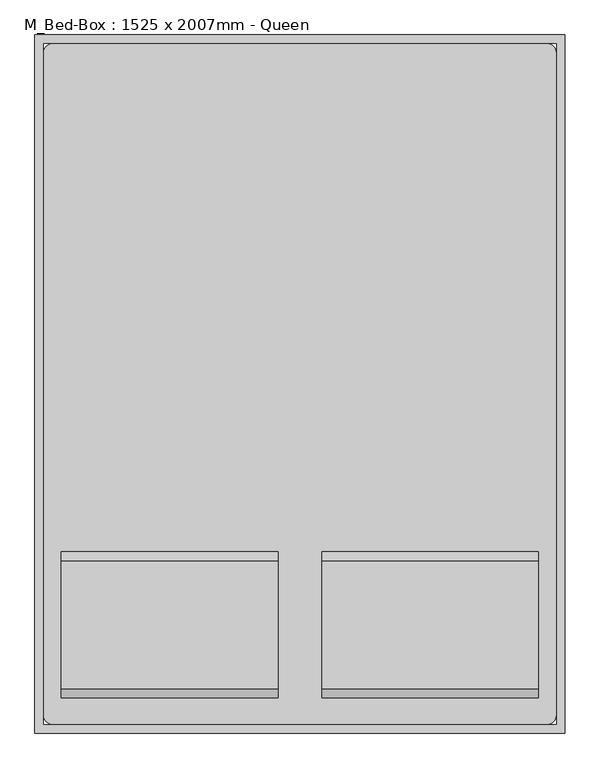
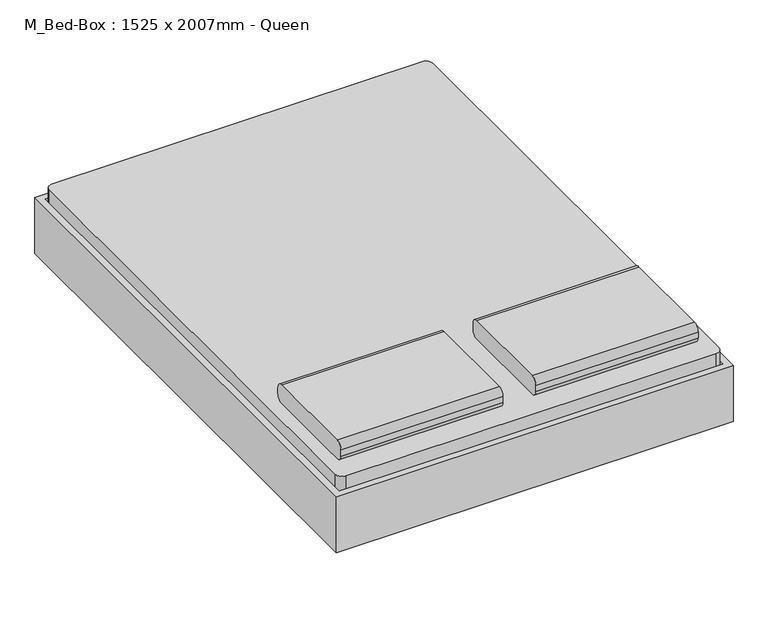
"""IFC4 building model written with IfcOpenShell, lengths in millimetres: furniture geometry, M_Bed-Box : 1525 x 2007mm - Queen."""

import ifcopenshell
import ifcopenshell.guid

model = None  # the IFC model being written
_history = None  # IfcOwnerHistory: only IFC2X3 demands one
_inside = {}  # id of a spatial element -> (the spatial element, [elements in it])
_under = {}  # id of a project, library or spatial element -> (it, [spatial elements below it])
_declared = {}  # id of a project -> (the project, [libraries it declares])
_typed = {}  # id of a type object -> (the type object, [elements of that type])
_made_of = {}  # id of a material, layer set ... -> (it, [elements and type objects made of it])


def new_model(schema):
    """Start an empty IFC model of exactly this schema.

    Asked for "IFC4X3", IfcOpenShell would pick the latest addendum, in which some entities
    have other attributes; the version numbers below select the first issue.
    IFC2X3 requires an IfcOwnerHistory on every rooted entity: one is made here for all.
    """
    global model, _history
    if schema == "IFC4X3":
        model = ifcopenshell.file(schema_version=(4, 3, 0, 0))
    else:
        model = ifcopenshell.file(schema=schema)
    _inside.clear()
    _under.clear()
    _declared.clear()
    _typed.clear()
    _made_of.clear()
    _history = None
    if model.schema == "IFC2X3":
        org = make("IfcOrganization", Name="unknown")
        user = make(
            "IfcPersonAndOrganization",
            ThePerson=make("IfcPerson", FamilyName="unknown"),
            TheOrganization=org,
        )
        app = make(
            "IfcApplication",
            ApplicationDeveloper=org,
            Version="unknown",
            ApplicationFullName="unknown",
            ApplicationIdentifier="unknown",
        )
        _history = make(
            "IfcOwnerHistory",
            OwningUser=user,
            OwningApplication=app,
            ChangeAction="ADDED",
            CreationDate=0,
        )
    return model


def make(cls, **values):
    """One entity of the class cls with the attributes given. An attribute that is None is left unset."""
    return model.create_entity(
        cls, **{name: value for name, value in values.items() if value is not None}
    )


def rooted(cls, **values):
    """An entity with a GlobalId (a new one), such as an element, a storey or a relation."""
    return make(cls, GlobalId=ifcopenshell.guid.new(), OwnerHistory=_history, **values)


def si_unit(unit_type, name, prefix=None):
    """IfcSIUnit, for example si_unit("LENGTHUNIT", "METRE", prefix="MILLI")."""
    return make("IfcSIUnit", UnitType=unit_type, Prefix=prefix, Name=name)


def assignment(units):
    """IfcUnitAssignment: the units of a project."""
    return None if units is None else make("IfcUnitAssignment", Units=units)


def point(xyz):
    """IfcCartesianPoint."""
    return None if xyz is None else make("IfcCartesianPoint", Coordinates=xyz)


def direction(xyz):
    """IfcDirection."""
    return None if xyz is None else make("IfcDirection", DirectionRatios=xyz)


def frame(location, z_axis=None, x_axis=None):
    """IfcAxis2Placement3D, a coordinate frame: its origin and axes. An axis left out is left unset."""
    return make(
        "IfcAxis2Placement3D",
        Location=point(location),
        Axis=direction(z_axis),
        RefDirection=direction(x_axis),
    )


def frame_2d(location, x_axis=None):
    """IfcAxis2Placement2D, a coordinate frame in the plane: its origin and x axis."""
    return make(
        "IfcAxis2Placement2D", Location=point(location), RefDirection=direction(x_axis)
    )


def origin():
    """The frame at (0, 0, 0) with its axes left unset."""
    return frame((0.0, 0.0, 0.0))


def place(relative_to, where):
    """IfcLocalPlacement: puts the frame where relative to a parent placement (None: the world)."""
    return make(
        "IfcLocalPlacement", PlacementRelTo=relative_to, RelativePlacement=where
    )


def context(
    kind, dimensions, precision=None, world=None, true_north=None, identifier=None
):
    """IfcGeometricRepresentationContext, for example the 3D "Model" context."""
    return make(
        "IfcGeometricRepresentationContext",
        ContextIdentifier=identifier,
        ContextType=kind,
        CoordinateSpaceDimension=dimensions,
        Precision=precision,
        WorldCoordinateSystem=world,
        TrueNorth=true_north,
    )


def project(units=None, contexts=None):
    """IfcProject with its units and contexts."""
    return rooted(
        "IfcProject",
        Name="project",
        RepresentationContexts=contexts,
        UnitsInContext=assignment(units),
    )


def spatial(cls, under=None, at=None, **own):
    """A site, building, storey or space (cls), placed at a placement, below another one or the project."""
    s = rooted(cls, ObjectPlacement=at, **own)
    if under is not None:
        _under.setdefault(under.id(), (under, []))[1].append(s)
    return s


def polyline(points):
    """IfcPolyline through the points."""
    return make("IfcPolyline", Points=[point(p) for p in points])


def circle_curve(where, radius):
    """IfcCircle in the frame where."""
    return make("IfcCircle", Position=where, Radius=radius)


def trimmed(basis, trim1, trim2, sense, master):
    """IfcTrimmedCurve: the piece of a basis curve between two trims."""
    return make(
        "IfcTrimmedCurve",
        BasisCurve=basis,
        Trim1=trim1,
        Trim2=trim2,
        SenseAgreement=sense,
        MasterRepresentation=master,
    )


def segment(curve, same_sense, transition):
    """IfcCompositeCurveSegment."""
    return make(
        "IfcCompositeCurveSegment",
        Transition=transition,
        SameSense=same_sense,
        ParentCurve=curve,
    )


def composite_curve(segments, self_intersect=None):
    """IfcCompositeCurve: segments joined end to end."""
    return make("IfcCompositeCurve", Segments=segments, SelfIntersect=self_intersect)


def outline(outer, holes=None, kind="AREA"):
    """IfcArbitraryClosedProfileDef: a profile drawn as a closed curve; with holes, ...WithVoids."""
    if holes is None:
        return make("IfcArbitraryClosedProfileDef", ProfileType=kind, OuterCurve=outer)
    return make(
        "IfcArbitraryProfileDefWithVoids",
        ProfileType=kind,
        OuterCurve=outer,
        InnerCurves=holes,
    )


def extrude(swept, where, along, depth):
    """IfcExtrudedAreaSolid: the profile swept, set in the frame where, extruded along a direction by depth."""
    return make(
        "IfcExtrudedAreaSolid",
        SweptArea=swept,
        Position=where,
        ExtrudedDirection=direction(along),
        Depth=depth,
    )


def shape(context_of_items, identifier, shape_type, items):
    """IfcShapeRepresentation: the items that make up one representation, for example the "Body"."""
    return make(
        "IfcShapeRepresentation",
        ContextOfItems=context_of_items,
        RepresentationIdentifier=identifier,
        RepresentationType=shape_type,
        Items=items,
    )


def source(mapping_origin, context_of_items, identifier, shape_type, items):
    """IfcRepresentationMap: a shape defined once, which mapped items show again and again."""
    return make(
        "IfcRepresentationMap",
        MappingOrigin=mapping_origin,
        MappedRepresentation=shape(context_of_items, identifier, shape_type, items),
    )


def transform(
    local_origin,
    x_axis=None,
    y_axis=None,
    z_axis=None,
    scale=None,
    scale2=None,
    scale3=None,
    uniform=True,
):
    """IfcCartesianTransformationOperator3D, or its non-uniform kind. x_axis, y_axis, z_axis: its Axis1, 2, 3."""
    if uniform:
        return make(
            "IfcCartesianTransformationOperator3D",
            Axis1=direction(x_axis),
            Axis2=direction(y_axis),
            LocalOrigin=point(local_origin),
            Scale=scale,
            Axis3=direction(z_axis),
        )
    return make(
        "IfcCartesianTransformationOperator3DnonUniform",
        Axis1=direction(x_axis),
        Axis2=direction(y_axis),
        LocalOrigin=point(local_origin),
        Scale=scale,
        Axis3=direction(z_axis),
        Scale2=scale2,
        Scale3=scale3,
    )


def mapped(mapping_source, mapping_target):
    """IfcMappedItem: shows the shape of a source again, moved by a transform."""
    return make(
        "IfcMappedItem", MappingSource=mapping_source, MappingTarget=mapping_target
    )


def made_of(thing, what):
    """Note that an element or type object is made of a material, layer set ...; save() writes the relation."""
    if what is not None:
        _made_of.setdefault(what.id(), (what, []))[1].append(thing)
    return thing


def element(
    cls,
    number,
    at=None,
    inside=None,
    cuts=None,
    type_object=None,
    material=None,
    context=None,
    identifier="Body",
    shape_type=None,
    held_by="IfcProductDefinitionShape",
    body=None,
    shapes=None,
    **own,
):
    """One element of the class cls, such as IfcWall. Its Tag is "e" and its number.

    at: its placement. inside: the storey or other place that contains it. cuts: it is an
    opening in that element (IfcRelVoidsElement). A single representation is given by context,
    identifier, shape_type and body (its items); several are given by shapes. held_by: the class
    of the entity that holds the representations. save() writes the other relations.
    """
    e = rooted(cls, Tag="e%d" % number, ObjectPlacement=at, **own)
    if body is not None:
        shapes = [shape(context, identifier, shape_type, body)]
    if shapes is not None:
        e.Representation = make(held_by, Representations=shapes)
    if inside is not None:
        _inside.setdefault(inside.id(), (inside, []))[1].append(e)
    if cuts is not None:
        rooted(
            "IfcRelVoidsElement", RelatingBuildingElement=cuts, RelatedOpeningElement=e
        )
    if type_object is not None:
        _typed.setdefault(type_object.id(), (type_object, []))[1].append(e)
    return made_of(e, material)


def aggregate(whole, parts):
    """IfcRelAggregates: a whole, such as a stair, and the parts it consists of."""
    return rooted("IfcRelAggregates", RelatingObject=whole, RelatedObjects=parts)


def save(model, path):
    """Write the relations noted so far, then the file.

    IfcRelAggregates (storeys below a building ...), IfcRelContainedInSpatialStructure (elements
    in a storey), IfcRelDefinesByType, IfcRelAssociatesMaterial and IfcRelDeclares: one each for
    every whole, place, type object, material and project.
    """
    for whole, parts in _under.values():
        aggregate(whole, parts)
    for where, things in _inside.values():
        rooted(
            "IfcRelContainedInSpatialStructure",
            RelatedElements=things,
            RelatingStructure=where,
        )
    for kind, things in _typed.values():
        rooted("IfcRelDefinesByType", RelatedObjects=things, RelatingType=kind)
    for what, things in _made_of.values():
        rooted("IfcRelAssociatesMaterial", RelatedObjects=things, RelatingMaterial=what)
    for by, libraries in _declared.values():
        rooted("IfcRelDeclares", RelatingContext=by, RelatedDefinitions=libraries)
    model.write(path)


def plane_surface(at):
    """IfcPlane: the flat surface through the origin of the frame at, square to its z axis."""
    return make("IfcPlane", Position=at)


def cylinder_surface(at, radius):
    """IfcCylindricalSurface: all points at the distance radius from the z axis of the frame at."""
    return make("IfcCylindricalSurface", Position=at, Radius=radius)


def revolved_surface(curve, axis_point, axis_direction):
    """IfcSurfaceOfRevolution: the curve turned about the line through axis_point along axis_direction."""
    return make(
        "IfcSurfaceOfRevolution",
        SweptCurve=make("IfcArbitraryOpenProfileDef", ProfileType="CURVE", Curve=curve),
        AxisPosition=make("IfcAxis1Placement", Location=point(axis_point), Axis=direction(axis_direction)),
    )


def advanced_brep(points, edges, surfaces, faces):
    """IfcAdvancedBrep: a solid bounded by faces that lie on surfaces and meet in shared edges.

    An edge is (start, end): straight between two places in points (the first is 0);
    or (start, end, curve); or (start, end, curve, False) where it runs against its curve.
    A face is (place in surfaces, loops), or (place, loops, False) where it looks against
    its surface's normal. A loop lists edges by number (the first is 1), with a minus sign
    where the edge is run from its end to its start. The first loop is the outer one.
    """
    corners = [point(p) for p in points]
    vertices = [make("IfcVertexPoint", VertexGeometry=c) for c in corners]
    made = []
    for start, end, *more in edges:
        made.append(
            make(
                "IfcEdgeCurve",
                EdgeStart=vertices[start],
                EdgeEnd=vertices[end],
                EdgeGeometry=more[0] if more else make("IfcPolyline", Points=[corners[start], corners[end]]),
                SameSense=more[1] if len(more) > 1 else True,
            )
        )
    hull = []
    for where, loops, *sense in faces:
        bounds = []
        for j, loop in enumerate(loops):
            ring = [make("IfcOrientedEdge", EdgeElement=made[abs(k) - 1], Orientation=k > 0) for k in loop]
            bounds.append(
                make(
                    "IfcFaceOuterBound" if j == 0 else "IfcFaceBound",
                    Bound=make("IfcEdgeLoop", EdgeList=ring),
                    Orientation=True,
                )
            )
        hull.append(make("IfcAdvancedFace", Bounds=bounds, FaceSurface=surfaces[where], SameSense=sense[0] if sense else True))
    return make("IfcAdvancedBrep", Outer=make("IfcClosedShell", CfsFaces=hull))


def m_bed_box_1525_x_2007mm_queen_6710bf5b(model_context):
    return source(origin(), model_context, "Body", "SolidModel", [
        extrude(outline(composite_curve([segment(trimmed(circle_curve(frame_2d((-642.0704918, 431.8)), 25.4), [point((-642.0704918, 406.4))], [point((-667.4704918, 431.8))], False, "CARTESIAN"), True, "CONTINUOUS"), segment(polyline([(-667.4704918, 431.8), (-667.4704918, 457.2)]), True, "CONTINUOUS"), segment(trimmed(circle_curve(frame_2d((-642.0704918, 457.2)), 25.4), [point((-667.4704918, 457.2))], [point((-642.0704918, 482.6))], False, "CARTESIAN"), True, "CONTINUOUS"), segment(polyline([(-642.0704918, 482.6), (-273.7704918, 482.6)]), True, "CONTINUOUS"), segment(trimmed(circle_curve(frame_2d((-273.7704918, 457.2)), 25.4), [point((-273.7704918, 482.6))], [point((-248.3704918, 457.2))], False, "CARTESIAN"), True, "CONTINUOUS"), segment(polyline([(-248.3704918, 457.2), (-248.3704918, 431.8)]), True, "CONTINUOUS"), segment(trimmed(circle_curve(frame_2d((-273.7704918, 431.8)), 25.4), [point((-248.3704918, 431.8))], [point((-273.7704918, 406.4))], False, "CARTESIAN"), True, "CONTINUOUS"), segment(polyline([(-273.7704918, 406.4), (-642.0704918, 406.4)]), True, "CONTINUOUS")], self_intersect=False)), frame((402.652459, 0.0, 0.0), z_axis=(1.0, 0.0, 0.0), x_axis=(0.0, 1.0, 0.0)), (0.0, 0.0, 1.0), 622.8),
        extrude(outline(composite_curve([segment(trimmed(circle_curve(frame_2d((-642.0704918, 431.8)), 25.4), [point((-642.0704918, 406.4))], [point((-667.4704918, 431.8))], False, "CARTESIAN"), True, "CONTINUOUS"), segment(polyline([(-667.4704918, 431.8), (-667.4704918, 457.2)]), True, "CONTINUOUS"), segment(trimmed(circle_curve(frame_2d((-642.0704918, 457.2)), 25.4), [point((-667.4704918, 457.2))], [point((-642.0704918, 482.6))], False, "CARTESIAN"), True, "CONTINUOUS"), segment(polyline([(-642.0704918, 482.6), (-273.7704918, 482.6)]), True, "CONTINUOUS"), segment(trimmed(circle_curve(frame_2d((-273.7704918, 457.2)), 25.4), [point((-273.7704918, 482.6))], [point((-248.3704918, 457.2))], False, "CARTESIAN"), True, "CONTINUOUS"), segment(polyline([(-248.3704918, 457.2), (-248.3704918, 431.8)]), True, "CONTINUOUS"), segment(trimmed(circle_curve(frame_2d((-273.7704918, 431.8)), 25.4), [point((-248.3704918, 431.8))], [point((-273.7704918, 406.4))], False, "CARTESIAN"), True, "CONTINUOUS"), segment(polyline([(-273.7704918, 406.4), (-642.0704918, 406.4)]), True, "CONTINUOUS")], self_intersect=False)), frame((-347.147541, 0.0, 0.0), z_axis=(1.0, 0.0, 0.0), x_axis=(0.0, 1.0, 0.0)), (0.0, 0.0, 1.0), 622.8),
        advanced_brep(
        [(-397.6231784, -515.0704918, 177.8), (-397.6231784, -515.0704918, 196.85), (-397.6231784, -438.8704918, 196.85), (-397.6231784, -438.8704918, 177.8), (-346.8231784, -438.8704918, 177.8), (-346.8231784, -515.0704918, 177.8), (-334.6869899, -438.8704918, 196.85), (-334.6869899, -515.0704918, 196.85), (-270.7523099, -438.8704918, 14.6654962), (-270.7523099, -515.0704918, 14.6654962), (-253.4871466, -438.8704918, 22.716374), (-253.4871466, -515.0704918, 22.716374), (-247.7320921, -438.8704918, 0.0), (-247.7320921, -515.0704918, 0.0), (-247.7320921, -438.8704918, 19.05), (-247.7320921, -515.0704918, 19.05), (-169.1195862, -438.8704918, 0.0), (-169.1195862, -515.0704918, 0.0), (-169.1195862, -438.8704918, 19.05), (-169.1195862, -515.0704918, 19.05), (-156.4195862, -438.8704918, 3.4029547), (-156.4195862, -515.0704918, 3.4029547), (-165.9445862, -438.8704918, 19.9007387), (-165.9445862, -515.0704918, 19.9007387), (-96.322541, -438.8704918, 38.1), (-96.322541, -515.0704918, 38.1), (-101.4269731, -438.8704918, 57.15), (-101.4269731, -515.0704918, 57.15), (774.9518216, -438.8704918, 38.1), (774.9518216, -515.0704918, 38.1), (780.0562537, -438.8704918, 57.15), (780.0562537, -515.0704918, 57.15), (835.0488669, -438.8704918, 3.4029547), (835.0488669, -515.0704918, 3.4029547), (844.5738669, -438.8704918, 19.9007387), (844.5738669, -515.0704918, 19.9007387), (847.7488669, -438.8704918, 0.0), (847.7488669, -515.0704918, 0.0), (847.7488669, -438.8704918, 19.05), (847.7488669, -515.0704918, 19.05), (926.3613728, -438.8704918, 0.0), (926.3613728, -515.0704918, 0.0), (926.3613728, -438.8704918, 19.05), (926.3613728, -515.0704918, 19.05), (949.3815906, -438.8704918, 14.6654962), (949.3815906, -515.0704918, 14.6654962), (932.1164272, -438.8704918, 22.716374), (932.1164272, -515.0704918, 22.716374), (1025.452459, -438.8704918, 177.8), (1025.452459, -515.0704918, 177.8), (1013.3162705, -438.8704918, 196.85), (1013.3162705, -515.0704918, 196.85), (1076.252459, -515.0704918, 177.8), (1076.252459, -438.8704918, 177.8), (1076.252459, -438.8704918, 196.85), (1076.252459, -515.0704918, 196.85)],
        [
            (0, 1),
            (1, 2),
            (2, 3),
            (3, 0),
            (3, 4),
            (4, 5),
            (5, 0),
            (2, 6),
            (6, 4),
            (1, 7),
            (7, 6),
            (5, 7),
            (4, 8),
            (8, 9),
            (9, 5),
            (6, 10),
            (10, 8),
            (7, 11),
            (11, 10),
            (9, 11),
            (12, 13),
            (13, 9, circle_curve(frame((-247.7320921, -515.0704918, 25.4), z_axis=(0.0, 1.0, 0.0), x_axis=(-0.906307787036649, 0.0, -0.4226182617407015)), 25.4)),
            (8, 12, circle_curve(frame((-247.7320921, -438.8704918, 25.4), z_axis=(0.0, -1.0, 0.0), x_axis=(-0.906307787036649, 0.0, -0.4226182617407015)), 25.4)),
            (14, 12),
            (10, 14, circle_curve(frame((-247.7320921, -438.8704918, 25.4), z_axis=(0.0, -1.0, 0.0), x_axis=(-0.906307787036649, 0.0, -0.4226182617407015)), 6.35)),
            (15, 14),
            (11, 15, circle_curve(frame((-247.7320921, -515.0704918, 25.4), z_axis=(0.0, -1.0, 0.0), x_axis=(-0.906307787036649, 0.0, -0.4226182617407015)), 6.35)),
            (13, 15),
            (12, 16),
            (16, 17),
            (17, 13),
            (14, 18),
            (18, 16),
            (15, 19),
            (19, 18),
            (17, 19),
            (20, 21),
            (21, 17, circle_curve(frame((-169.1195862, -515.0704918, 25.4), z_axis=(0.0, 1.0, 0.0), x_axis=(0.0, 0.0, -1.0)), 25.4)),
            (16, 20, circle_curve(frame((-169.1195862, -438.8704918, 25.4), z_axis=(0.0, -1.0, 0.0), x_axis=(0.0, 0.0, -1.0)), 25.4)),
            (22, 20),
            (18, 22, circle_curve(frame((-169.1195862, -438.8704918, 25.4), z_axis=(0.0, -1.0, 0.0), x_axis=(0.0, 0.0, -1.0)), 6.35)),
            (23, 22),
            (19, 23, circle_curve(frame((-169.1195862, -515.0704918, 25.4), z_axis=(0.0, -1.0, 0.0), x_axis=(0.0, 0.0, -1.0)), 6.35)),
            (21, 23),
            (20, 24),
            (24, 25),
            (25, 21),
            (22, 26),
            (26, 24),
            (23, 27),
            (27, 26),
            (25, 27),
            (24, 28),
            (28, 29),
            (29, 25),
            (26, 30),
            (30, 28),
            (27, 31),
            (31, 30),
            (29, 31),
            (28, 32),
            (32, 33),
            (33, 29),
            (30, 34),
            (34, 32),
            (31, 35),
            (35, 34),
            (33, 35),
            (36, 37),
            (37, 33, circle_curve(frame((847.7488669, -515.0704918, 25.4), z_axis=(0.0, 1.0, 0.0), x_axis=(-0.5000000000000463, 0.0, -0.8660254037844118)), 25.4)),
            (32, 36, circle_curve(frame((847.7488669, -438.8704918, 25.4), z_axis=(0.0, -1.0, 0.0), x_axis=(-0.5000000000000463, 0.0, -0.8660254037844118)), 25.4)),
            (38, 36),
            (34, 38, circle_curve(frame((847.7488669, -438.8704918, 25.4), z_axis=(0.0, -1.0, 0.0), x_axis=(-0.5000000000000463, 0.0, -0.8660254037844118)), 6.35)),
            (39, 38),
            (35, 39, circle_curve(frame((847.7488669, -515.0704918, 25.4), z_axis=(0.0, -1.0, 0.0), x_axis=(-0.5000000000000463, 0.0, -0.8660254037844118)), 6.35)),
            (37, 39),
            (36, 40),
            (40, 41),
            (41, 37),
            (38, 42),
            (42, 40),
            (39, 43),
            (43, 42),
            (41, 43),
            (44, 45),
            (45, 41, circle_curve(frame((926.3613728, -515.0704918, 25.4), z_axis=(0.0, 1.0, 0.0), x_axis=(0.0, 0.0, -1.0)), 25.4)),
            (40, 44, circle_curve(frame((926.3613728, -438.8704918, 25.4), z_axis=(0.0, -1.0, 0.0), x_axis=(0.0, 0.0, -1.0)), 25.4)),
            (46, 44),
            (42, 46, circle_curve(frame((926.3613728, -438.8704918, 25.4), z_axis=(0.0, -1.0, 0.0), x_axis=(0.0, 0.0, -1.0)), 6.35)),
            (47, 46),
            (43, 47, circle_curve(frame((926.3613728, -515.0704918, 25.4), z_axis=(0.0, -1.0, 0.0), x_axis=(0.0, 0.0, -1.0)), 6.35)),
            (45, 47),
            (44, 48),
            (48, 49),
            (49, 45),
            (46, 50),
            (50, 48),
            (47, 51),
            (51, 50),
            (49, 51),
            (52, 53),
            (53, 54),
            (54, 55),
            (55, 52),
            (48, 53),
            (52, 49),
            (50, 54),
            (51, 55),
        ],
        [
            plane_surface(frame((-397.6231784, -769.0704918, -152.9490627), z_axis=(-1.0, 0.0, 0.0), x_axis=(0.0, -1.0, 0.0))),
            plane_surface(frame((-397.6231784, -515.0704918, 177.8), z_axis=(0.0, 0.0, -1.0), x_axis=(1.0, 0.0, 0.0))),
            plane_surface(frame((-397.6231784, -438.8704918, 177.8), z_axis=(0.0, 1.0, 0.0), x_axis=(1.0, 0.0, 0.0))),
            plane_surface(frame((-397.6231784, -438.8704918, 196.85), z_axis=(0.0, 0.0, 1.0), x_axis=(1.0, 0.0, 0.0))),
            plane_surface(frame((-397.6231784, -515.0704918, 196.85), z_axis=(0.0, -1.0, 0.0), x_axis=(1.0, 0.0, 0.0))),
            plane_surface(frame((-346.8231784, -515.0704918, 177.8), z_axis=(-0.9063077870366485, 0.0, -0.4226182617407029), x_axis=(0.4226182617407029, 0.0, -0.9063077870366485))),
            plane_surface(frame((-346.8231784, -438.8704918, 177.8), z_axis=(0.0, 1.0, 0.0), x_axis=(0.42261826174070266, 0.0, -0.9063077870366485))),
            plane_surface(frame((-334.6869899, -438.8704918, 196.85), z_axis=(0.9063077870366486, 0.0, 0.4226182617407026), x_axis=(0.4226182617407026, 0.0, -0.9063077870366486))),
            plane_surface(frame((-334.6869899, -515.0704918, 196.85), z_axis=(0.0, -1.0, 0.0), x_axis=(0.42261826174070266, 0.0, -0.9063077870366485))),
            cylinder_surface(frame((-247.7320921, -769.0704918, 25.4), z_axis=(0.0, 1.0, 0.0), x_axis=(-0.906307787036649, 0.0, -0.4226182617407015)), 25.4),
            plane_surface(frame((-247.7320921, -438.8704918, 25.4), z_axis=(0.0, 1.0, 0.0), x_axis=(-0.906307787036649, 0.0, -0.4226182617407015))),
            revolved_surface(polyline([(-253.4871465476827, -438.8704918, 22.716374037946544), (-253.4871465476827, -515.0704918, 22.716374037946544)]), (-247.7320921, -769.0704918, 25.4), (0.0, 1.0, 0.0)),
            plane_surface(frame((-247.7320921, -515.0704918, 25.4), z_axis=(0.0, -1.0, 0.0), x_axis=(-0.906307787036649, 0.0, -0.4226182617407015))),
            plane_surface(frame((-247.7320921, -515.0704918, 0.0), z_axis=(0.0, 0.0, -1.0), x_axis=(1.0, 0.0, 0.0))),
            plane_surface(frame((-247.7320921, -438.8704918, 0.0), z_axis=(0.0, 1.0, 0.0), x_axis=(1.0, 0.0, 0.0))),
            plane_surface(frame((-247.7320921, -438.8704918, 19.05), z_axis=(0.0, 0.0, 1.0), x_axis=(1.0, 0.0, 0.0))),
            plane_surface(frame((-247.7320921, -515.0704918, 19.05), z_axis=(0.0, -1.0, 0.0), x_axis=(1.0, 0.0, 0.0))),
            cylinder_surface(frame((-169.1195862, -769.0704918, 25.4), z_axis=(0.0, 1.0, 0.0), x_axis=(0.0, 0.0, -1.0)), 25.4),
            plane_surface(frame((-169.1195862, -438.8704918, 25.4), z_axis=(0.0, 1.0, 0.0), x_axis=(0.0, 0.0, -1.0))),
            revolved_surface(polyline([(-169.1195862, -438.8704918, 19.049999999999997), (-169.1195862, -515.0704918, 19.049999999999997)]), (-169.1195862, -769.0704918, 25.4), (0.0, 1.0, 0.0)),
            plane_surface(frame((-169.1195862, -515.0704918, 25.4), z_axis=(0.0, -1.0, 0.0), x_axis=(0.0, 0.0, -1.0))),
            plane_surface(frame((-156.4195862, -515.0704918, 3.4029547), z_axis=(0.49999999999987765, 0.0, -0.8660254037845093), x_axis=(0.8660254037845093, 0.0, 0.49999999999987765))),
            plane_surface(frame((-156.4195862, -438.8704918, 3.4029547), z_axis=(0.0, 1.0, 0.0), x_axis=(0.8660254037845091, 0.0, 0.499999999999878))),
            plane_surface(frame((-165.9445862, -438.8704918, 19.9007387), z_axis=(-0.49999999999987765, 0.0, 0.8660254037845093), x_axis=(0.8660254037845093, 0.0, 0.49999999999987765))),
            plane_surface(frame((-165.9445862, -515.0704918, 19.9007387), z_axis=(0.0, -1.0000000000000002, 0.0), x_axis=(0.8660254037845089, 0.0, 0.4999999999998785))),
            plane_surface(frame((-96.322541, -515.0704918, 38.1), z_axis=(0.0, 0.0, -1.0), x_axis=(1.0, 0.0, 0.0))),
            plane_surface(frame((-96.322541, -438.8704918, 38.1), z_axis=(0.0, 1.0, 0.0), x_axis=(1.0, 0.0, 0.0))),
            plane_surface(frame((-101.4269731, -438.8704918, 57.15), z_axis=(0.0, 0.0, 1.0), x_axis=(1.0, 0.0, 0.0))),
            plane_surface(frame((-101.4269731, -515.0704918, 57.15), z_axis=(0.0, -1.0, 0.0), x_axis=(1.0, 0.0, 0.0))),
            plane_surface(frame((774.9518216, -515.0704918, 38.1), z_axis=(-0.5000000000000452, 0.0, -0.8660254037844126), x_axis=(0.8660254037844126, 0.0, -0.5000000000000452))),
            plane_surface(frame((774.9518216, -438.8704918, 38.1), z_axis=(0.0, 1.0, 0.0), x_axis=(0.8660254037844124, 0.0, -0.5000000000000455))),
            plane_surface(frame((780.0562537, -438.8704918, 57.15), z_axis=(0.5000000000000464, 0.0, 0.8660254037844118), x_axis=(0.8660254037844118, 0.0, -0.5000000000000464))),
            plane_surface(frame((780.0562537, -515.0704918, 57.15), z_axis=(0.0, -1.0000000000000002, 0.0), x_axis=(0.866025403784413, 0.0, -0.5000000000000447))),
            cylinder_surface(frame((847.7488669, -769.0704918, 25.4), z_axis=(0.0, 1.0, 0.0), x_axis=(-0.5000000000000463, 0.0, -0.8660254037844118)), 25.4),
            plane_surface(frame((847.7488669, -438.8704918, 25.4), z_axis=(0.0, 1.0000000000000002, 0.0), x_axis=(-0.5000000000000464, 0.0, -0.866025403784412))),
            revolved_surface(polyline([(844.5738668999998, -438.8704918, 19.90073868596898), (844.5738668999998, -515.0704918, 19.90073868596898)]), (847.7488669, -769.0704918, 25.4), (0.0, 1.0, 0.0)),
            plane_surface(frame((847.7488669, -515.0704918, 25.4), z_axis=(0.0, -1.0000000000000002, 0.0), x_axis=(-0.5000000000000464, 0.0, -0.866025403784412))),
            plane_surface(frame((847.7488669, -515.0704918, 0.0), z_axis=(0.0, 0.0, -1.0), x_axis=(1.0, 0.0, 0.0))),
            plane_surface(frame((847.7488669, -438.8704918, 0.0), z_axis=(0.0, 1.0, 0.0), x_axis=(1.0, 0.0, 0.0))),
            plane_surface(frame((847.7488669, -438.8704918, 19.05), z_axis=(0.0, 0.0, 1.0), x_axis=(1.0, 0.0, 0.0))),
            plane_surface(frame((847.7488669, -515.0704918, 19.05), z_axis=(0.0, -1.0, 0.0), x_axis=(1.0, 0.0, 0.0))),
            cylinder_surface(frame((926.3613728, -769.0704918, 25.4), z_axis=(0.0, 1.0, 0.0), x_axis=(0.0, 0.0, -1.0)), 25.4),
            plane_surface(frame((926.3613728, -438.8704918, 25.4), z_axis=(0.0, 1.0, 0.0), x_axis=(0.0, 0.0, -1.0))),
            revolved_surface(polyline([(926.3613728, -438.8704918, 19.049999999999997), (926.3613728, -515.0704918, 19.049999999999997)]), (926.3613728, -769.0704918, 25.4), (0.0, 1.0, 0.0)),
            plane_surface(frame((926.3613728, -515.0704918, 25.4), z_axis=(0.0, -1.0, 0.0), x_axis=(0.0, 0.0, -1.0))),
            plane_surface(frame((949.3815906, -515.0704918, 14.6654962), z_axis=(0.9063077870366805, 0.0, -0.422618261740634), x_axis=(0.422618261740634, 0.0, 0.9063077870366805))),
            plane_surface(frame((949.3815906, -438.8704918, 14.6654962), z_axis=(0.0, 1.0, 0.0), x_axis=(0.4226182617406339, 0.0, 0.9063077870366806))),
            plane_surface(frame((932.1164272, -438.8704918, 22.716374), z_axis=(-0.9063077870366808, 0.0, 0.4226182617406335), x_axis=(0.4226182617406335, 0.0, 0.9063077870366808))),
            plane_surface(frame((932.1164272, -515.0704918, 22.716374), z_axis=(0.0, -1.0, 0.0), x_axis=(0.42261826174063294, 0.0, 0.906307787036681))),
            plane_surface(frame((1076.252459, -769.0704918, -152.9490627), z_axis=(1.0, 0.0, 0.0), x_axis=(0.0, -1.0, 0.0))),
            plane_surface(frame((1025.452459, -515.0704918, 177.8), z_axis=(0.0, 0.0, -1.0), x_axis=(1.0, 0.0, 0.0))),
            plane_surface(frame((1025.452459, -438.8704918, 177.8), z_axis=(0.0, 1.0, 0.0), x_axis=(1.0, 0.0, 0.0))),
            plane_surface(frame((1013.3162705, -438.8704918, 196.85), z_axis=(0.0, 0.0, 1.0), x_axis=(1.0, 0.0, 0.0))),
            plane_surface(frame((1013.3162705, -515.0704918, 196.85), z_axis=(0.0, -1.0, 0.0), x_axis=(1.0, 0.0, 0.0))),
        ],
        [
            (0, [[1, 2, 3, 4]]),
            (1, [[5, 6, 7, -4]]),
            (2, [[8, 9, -5, -3]]),
            (3, [[10, 11, -8, -2]]),
            (4, [[-7, 12, -10, -1]]),
            (5, [[13, 14, 15, -6]]),
            (6, [[16, 17, -13, -9]]),
            (7, [[18, 19, -16, -11]]),
            (8, [[-15, 20, -18, -12]]),
            (9, [[21, 22, -14, 23]]),
            (10, [[24, -23, -17, 25]]),
            (11, [[26, -25, -19, 27]]),
            (12, [[28, -27, -20, -22]]),
            (13, [[29, 30, 31, -21]]),
            (14, [[32, 33, -29, -24]]),
            (15, [[34, 35, -32, -26]]),
            (16, [[-31, 36, -34, -28]]),
            (17, [[37, 38, -30, 39]]),
            (18, [[40, -39, -33, 41]]),
            (19, [[42, -41, -35, 43]]),
            (20, [[44, -43, -36, -38]]),
            (21, [[45, 46, 47, -37]]),
            (22, [[48, 49, -45, -40]]),
            (23, [[50, 51, -48, -42]]),
            (24, [[-47, 52, -50, -44]]),
            (25, [[53, 54, 55, -46]]),
            (26, [[56, 57, -53, -49]]),
            (27, [[58, 59, -56, -51]]),
            (28, [[-55, 60, -58, -52]]),
            (29, [[61, 62, 63, -54]]),
            (30, [[64, 65, -61, -57]]),
            (31, [[66, 67, -64, -59]]),
            (32, [[-63, 68, -66, -60]]),
            (33, [[69, 70, -62, 71]]),
            (34, [[72, -71, -65, 73]]),
            (35, [[74, -73, -67, 75]]),
            (36, [[76, -75, -68, -70]]),
            (37, [[77, 78, 79, -69]]),
            (38, [[80, 81, -77, -72]]),
            (39, [[82, 83, -80, -74]]),
            (40, [[-79, 84, -82, -76]]),
            (41, [[85, 86, -78, 87]]),
            (42, [[88, -87, -81, 89]]),
            (43, [[90, -89, -83, 91]]),
            (44, [[92, -91, -84, -86]]),
            (45, [[93, 94, 95, -85]]),
            (46, [[96, 97, -93, -88]]),
            (47, [[98, 99, -96, -90]]),
            (48, [[-95, 100, -98, -92]]),
            (49, [[101, 102, 103, 104]]),
            (50, [[105, -101, 106, -94]]),
            (51, [[107, -102, -105, -97]]),
            (52, [[108, -103, -107, -99]]),
            (53, [[-106, -104, -108, -100]]),
        ],
    ),
        extrude(outline(composite_curve([segment(trimmed(circle_curve(frame_2d((-372.547541, -718.2704918)), 25.4), [point((-372.547541, -743.6704918))], [point((-397.947541, -718.2704918))], False, "CARTESIAN"), True, "CONTINUOUS"), segment(polyline([(-397.947541, -718.2704918), (-397.947541, 1187.1295082)]), True, "CONTINUOUS"), segment(trimmed(circle_curve(frame_2d((-372.547541, 1187.1295082)), 25.4), [point((-397.947541, 1187.1295082))], [point((-372.547541, 1212.5295082))], False, "CARTESIAN"), True, "CONTINUOUS"), segment(polyline([(-372.547541, 1212.5295082), (1050.852459, 1212.5295082)]), True, "CONTINUOUS"), segment(trimmed(circle_curve(frame_2d((1050.852459, 1187.1295082)), 25.4), [point((1050.852459, 1212.5295082))], [point((1076.252459, 1187.1295082))], False, "CARTESIAN"), True, "CONTINUOUS"), segment(polyline([(1076.252459, 1187.1295082), (1076.252459, -718.2704918)]), True, "CONTINUOUS"), segment(trimmed(circle_curve(frame_2d((1050.852459, -718.2704918)), 25.4), [point((1076.252459, -718.2704918))], [point((1050.852459, -743.6704918))], False, "CARTESIAN"), True, "CONTINUOUS"), segment(polyline([(1050.852459, -743.6704918), (-372.547541, -743.6704918)]), True, "CONTINUOUS")], self_intersect=False)), frame((0.0, 0.0, 203.2), z_axis=(0.0, 0.0, 1.0), x_axis=(1.0, 0.0, 0.0)), (0.0, 0.0, 1.0), 203.2),
        advanced_brep(
        [(-397.947541, 933.1295082, 196.85), (-397.947541, 1009.3295082, 196.85), (-397.947541, 1009.3295082, 177.8), (-397.947541, 933.1295082, 177.8), (-347.147541, 933.1295082, 177.8), (-335.0113525, 933.1295082, 196.85), (-347.147541, 1009.3295082, 177.8), (-335.0113525, 1009.3295082, 196.85), (-271.0766725, 933.1295082, 14.6654962), (-253.8115092, 933.1295082, 22.716374), (-271.0766725, 1009.3295082, 14.6654962), (-253.8115092, 1009.3295082, 22.716374), (-248.0564547, 933.1295082, 0.0), (-248.0564547, 933.1295082, 19.05), (-248.0564547, 1009.3295082, 0.0), (-248.0564547, 1009.3295082, 19.05), (-169.4439489, 933.1295082, 0.0), (-169.4439489, 933.1295082, 19.05), (-169.4439489, 1009.3295082, 0.0), (-169.4439489, 1009.3295082, 19.05), (-156.7439489, 933.1295082, 3.4029547), (-166.2689489, 933.1295082, 19.9007387), (-156.7439489, 1009.3295082, 3.4029547), (-166.2689489, 1009.3295082, 19.9007387), (-96.6469036, 933.1295082, 38.1), (-101.7513357, 933.1295082, 57.15), (-96.6469036, 1009.3295082, 38.1), (-101.7513357, 1009.3295082, 57.15), (774.9518216, 933.1295082, 38.1), (780.0562537, 933.1295082, 57.15), (774.9518216, 1009.3295082, 38.1), (780.0562537, 1009.3295082, 57.15), (835.0488669, 933.1295082, 3.4029547), (844.5738669, 933.1295082, 19.9007387), (835.0488669, 1009.3295082, 3.4029547), (844.5738669, 1009.3295082, 19.9007387), (847.7488669, 933.1295082, 0.0), (847.7488669, 933.1295082, 19.05), (847.7488669, 1009.3295082, 0.0), (847.7488669, 1009.3295082, 19.05), (926.3613728, 933.1295082, 0.0), (926.3613728, 933.1295082, 19.05), (926.3613728, 1009.3295082, 0.0), (926.3613728, 1009.3295082, 19.05), (949.3815906, 933.1295082, 14.6654962), (932.1164272, 933.1295082, 22.716374), (949.3815906, 1009.3295082, 14.6654962), (932.1164272, 1009.3295082, 22.716374), (1025.452459, 933.1295082, 177.8), (1013.3162705, 933.1295082, 196.85), (1025.452459, 1009.3295082, 177.8), (1013.3162705, 1009.3295082, 196.85), (1076.252459, 933.1295082, 196.85), (1076.252459, 933.1295082, 177.8), (1076.252459, 1009.3295082, 177.8), (1076.252459, 1009.3295082, 196.85)],
        [
            (0, 1),
            (1, 2),
            (2, 3),
            (3, 0),
            (3, 4),
            (4, 5),
            (5, 0),
            (2, 6),
            (6, 4),
            (1, 7),
            (7, 6),
            (5, 7),
            (4, 8),
            (8, 9),
            (9, 5),
            (6, 10),
            (10, 8),
            (7, 11),
            (11, 10),
            (9, 11),
            (12, 13),
            (13, 9, circle_curve(frame((-248.0564547, 933.1295082, 25.4), z_axis=(0.0, 1.0, 0.0), x_axis=(-0.9063077870366625, 0.0, -0.4226182617406725)), 6.35)),
            (8, 12, circle_curve(frame((-248.0564547, 933.1295082, 25.4), z_axis=(0.0, -1.0, 0.0), x_axis=(-0.9063077870366625, 0.0, -0.4226182617406725)), 25.4)),
            (14, 12),
            (10, 14, circle_curve(frame((-248.0564547, 1009.3295082, 25.4), z_axis=(0.0, -1.0, 0.0), x_axis=(-0.9063077870366625, 0.0, -0.4226182617406725)), 25.4)),
            (15, 14),
            (11, 15, circle_curve(frame((-248.0564547, 1009.3295082, 25.4), z_axis=(0.0, -1.0, 0.0), x_axis=(-0.9063077870366625, 0.0, -0.4226182617406725)), 6.35)),
            (13, 15),
            (12, 16),
            (16, 17),
            (17, 13),
            (14, 18),
            (18, 16),
            (15, 19),
            (19, 18),
            (17, 19),
            (20, 21),
            (21, 17, circle_curve(frame((-169.4439489, 933.1295082, 25.4), z_axis=(0.0, 1.0, 0.0), x_axis=(0.0, 0.0, -1.0)), 6.35)),
            (16, 20, circle_curve(frame((-169.4439489, 933.1295082, 25.4), z_axis=(0.0, -1.0, 0.0), x_axis=(0.0, 0.0, -1.0)), 25.4)),
            (22, 20),
            (18, 22, circle_curve(frame((-169.4439489, 1009.3295082, 25.4), z_axis=(0.0, -1.0, 0.0), x_axis=(0.0, 0.0, -1.0)), 25.4)),
            (23, 22),
            (19, 23, circle_curve(frame((-169.4439489, 1009.3295082, 25.4), z_axis=(0.0, -1.0, 0.0), x_axis=(0.0, 0.0, -1.0)), 6.35)),
            (21, 23),
            (20, 24),
            (24, 25),
            (25, 21),
            (22, 26),
            (26, 24),
            (23, 27),
            (27, 26),
            (25, 27),
            (24, 28),
            (28, 29),
            (29, 25),
            (26, 30),
            (30, 28),
            (27, 31),
            (31, 30),
            (29, 31),
            (28, 32),
            (32, 33),
            (33, 29),
            (30, 34),
            (34, 32),
            (31, 35),
            (35, 34),
            (33, 35),
            (36, 37),
            (37, 33, circle_curve(frame((847.7488669, 933.1295082, 25.4), z_axis=(0.0, 1.0, 0.0), x_axis=(-0.5000000000000528, 0.0, -0.8660254037844081)), 6.35)),
            (32, 36, circle_curve(frame((847.7488669, 933.1295082, 25.4), z_axis=(0.0, -1.0, 0.0), x_axis=(-0.5000000000000528, 0.0, -0.8660254037844081)), 25.4)),
            (38, 36),
            (34, 38, circle_curve(frame((847.7488669, 1009.3295082, 25.4), z_axis=(0.0, -1.0, 0.0), x_axis=(-0.5000000000000528, 0.0, -0.8660254037844081)), 25.4)),
            (39, 38),
            (35, 39, circle_curve(frame((847.7488669, 1009.3295082, 25.4), z_axis=(0.0, -1.0, 0.0), x_axis=(-0.5000000000000528, 0.0, -0.8660254037844081)), 6.35)),
            (37, 39),
            (36, 40),
            (40, 41),
            (41, 37),
            (38, 42),
            (42, 40),
            (39, 43),
            (43, 42),
            (41, 43),
            (44, 45),
            (45, 41, circle_curve(frame((926.3613728, 933.1295082, 25.4), z_axis=(0.0, 1.0, 0.0), x_axis=(0.0, 0.0, -1.0)), 6.35)),
            (40, 44, circle_curve(frame((926.3613728, 933.1295082, 25.4), z_axis=(0.0, -1.0, 0.0), x_axis=(0.0, 0.0, -1.0)), 25.4)),
            (46, 44),
            (42, 46, circle_curve(frame((926.3613728, 1009.3295082, 25.4), z_axis=(0.0, -1.0, 0.0), x_axis=(0.0, 0.0, -1.0)), 25.4)),
            (47, 46),
            (43, 47, circle_curve(frame((926.3613728, 1009.3295082, 25.4), z_axis=(0.0, -1.0, 0.0), x_axis=(0.0, 0.0, -1.0)), 6.35)),
            (45, 47),
            (44, 48),
            (48, 49),
            (49, 45),
            (46, 50),
            (50, 48),
            (47, 51),
            (51, 50),
            (49, 51),
            (52, 53),
            (53, 54),
            (54, 55),
            (55, 52),
            (48, 53),
            (52, 49),
            (50, 54),
            (51, 55),
        ],
        [
            plane_surface(frame((-397.947541, 1237.9295082, -127.5947323), z_axis=(-1.0, 0.0, 0.0), x_axis=(0.0, -1.0, 0.0))),
            plane_surface(frame((-397.947541, 933.1295082, 196.85), z_axis=(0.0, -1.0, 0.0), x_axis=(1.0, 0.0, 0.0))),
            plane_surface(frame((-397.947541, 933.1295082, 177.8), z_axis=(0.0, 0.0, -1.0), x_axis=(1.0, 0.0, 0.0))),
            plane_surface(frame((-397.947541, 1009.3295082, 177.8), z_axis=(0.0, 1.0, 0.0), x_axis=(1.0, 0.0, 0.0))),
            plane_surface(frame((-397.947541, 1009.3295082, 196.85), z_axis=(0.0, 0.0, 1.0), x_axis=(1.0, 0.0, 0.0))),
            plane_surface(frame((-335.0113525, 933.1295082, 196.85), z_axis=(0.0, -1.0, 0.0), x_axis=(0.42261826174067124, 0.0, -0.9063077870366631))),
            plane_surface(frame((-347.147541, 933.1295082, 177.8), z_axis=(-0.9063077870366631, 0.0, -0.42261826174067113), x_axis=(0.42261826174067113, 0.0, -0.9063077870366631))),
            plane_surface(frame((-347.147541, 1009.3295082, 177.8), z_axis=(0.0, 1.0, 0.0), x_axis=(0.422618261740671, 0.0, -0.9063077870366633))),
            plane_surface(frame((-335.0113525, 1009.3295082, 196.85), z_axis=(0.9063077870366631, 0.0, 0.42261826174067124), x_axis=(0.42261826174067124, 0.0, -0.9063077870366631))),
            plane_surface(frame((-248.0564547, 933.1295082, 25.4), z_axis=(0.0, -1.0, 0.0), x_axis=(-0.9063077870366625, 0.0, -0.4226182617406725))),
            cylinder_surface(frame((-248.0564547, 1237.9295082, 25.4), z_axis=(0.0, 1.0, 0.0), x_axis=(-0.9063077870366625, 0.0, -0.4226182617406725)), 25.4),
            plane_surface(frame((-248.0564547, 1009.3295082, 25.4), z_axis=(0.0, 1.0, 0.0), x_axis=(-0.9063077870366625, 0.0, -0.4226182617406725))),
            revolved_surface(polyline([(-253.81150914768278, 1009.3295082, 22.71637403794673), (-253.81150914768278, 933.1295082, 22.71637403794673)]), (-248.0564547, 1237.9295082, 25.4), (0.0, 1.0, 0.0)),
            plane_surface(frame((-248.0564547, 933.1295082, 19.05), z_axis=(0.0, -1.0, 0.0), x_axis=(1.0, 0.0, 0.0))),
            plane_surface(frame((-248.0564547, 933.1295082, 0.0), z_axis=(0.0, 0.0, -1.0), x_axis=(1.0, 0.0, 0.0))),
            plane_surface(frame((-248.0564547, 1009.3295082, 0.0), z_axis=(0.0, 1.0, 0.0), x_axis=(1.0, 0.0, 0.0))),
            plane_surface(frame((-248.0564547, 1009.3295082, 19.05), z_axis=(0.0, 0.0, 1.0), x_axis=(1.0, 0.0, 0.0))),
            plane_surface(frame((-169.4439489, 933.1295082, 25.4), z_axis=(0.0, -1.0, 0.0), x_axis=(0.0, 0.0, -1.0))),
            cylinder_surface(frame((-169.4439489, 1237.9295082, 25.4), z_axis=(0.0, 1.0, 0.0), x_axis=(0.0, 0.0, -1.0)), 25.4),
            plane_surface(frame((-169.4439489, 1009.3295082, 25.4), z_axis=(0.0, 1.0, 0.0), x_axis=(0.0, 0.0, -1.0))),
            revolved_surface(polyline([(-169.4439489, 1009.3295082, 19.049999999999997), (-169.4439489, 933.1295082, 19.049999999999997)]), (-169.4439489, 1237.9295082, 25.4), (0.0, 1.0, 0.0)),
            plane_surface(frame((-166.2689489, 933.1295082, 19.9007387), z_axis=(0.0, -1.0, 0.0), x_axis=(0.8660254037844788, 0.0, 0.49999999999993056))),
            plane_surface(frame((-156.7439489, 933.1295082, 3.4029547), z_axis=(0.4999999999999305, 0.0, -0.8660254037844788), x_axis=(0.8660254037844788, 0.0, 0.4999999999999305))),
            plane_surface(frame((-156.7439489, 1009.3295082, 3.4029547), z_axis=(0.0, 1.0, 0.0), x_axis=(0.8660254037844788, 0.0, 0.49999999999993044))),
            plane_surface(frame((-166.2689489, 1009.3295082, 19.9007387), z_axis=(-0.49999999999993033, 0.0, 0.8660254037844789), x_axis=(0.8660254037844789, 0.0, 0.49999999999993033))),
            plane_surface(frame((-101.7513357, 933.1295082, 57.15), z_axis=(0.0, -1.0, 0.0), x_axis=(1.0, 0.0, 0.0))),
            plane_surface(frame((-96.6469036, 933.1295082, 38.1), z_axis=(0.0, 0.0, -1.0), x_axis=(1.0, 0.0, 0.0))),
            plane_surface(frame((-96.6469036, 1009.3295082, 38.1), z_axis=(0.0, 1.0, 0.0), x_axis=(1.0, 0.0, 0.0))),
            plane_surface(frame((-101.7513357, 1009.3295082, 57.15), z_axis=(0.0, 0.0, 1.0), x_axis=(1.0, 0.0, 0.0))),
            plane_surface(frame((780.0562537, 933.1295082, 57.15), z_axis=(0.0, -1.0, 0.0), x_axis=(0.8660254037844092, 0.0, -0.5000000000000511))),
            plane_surface(frame((774.9518216, 933.1295082, 38.1), z_axis=(-0.5000000000000514, 0.0, -0.866025403784409), x_axis=(0.866025403784409, 0.0, -0.5000000000000514))),
            plane_surface(frame((774.9518216, 1009.3295082, 38.1), z_axis=(0.0, 1.0, 0.0), x_axis=(0.8660254037844092, 0.0, -0.5000000000000512))),
            plane_surface(frame((780.0562537, 1009.3295082, 57.15), z_axis=(0.500000000000051, 0.0, 0.8660254037844093), x_axis=(0.8660254037844093, 0.0, -0.500000000000051))),
            plane_surface(frame((847.7488669, 933.1295082, 25.4), z_axis=(0.0, -1.0000000000000002, 0.0), x_axis=(-0.500000000000053, 0.0, -0.8660254037844082))),
            cylinder_surface(frame((847.7488669, 1237.9295082, 25.4), z_axis=(0.0, 1.0, 0.0), x_axis=(-0.5000000000000528, 0.0, -0.8660254037844081)), 25.4),
            plane_surface(frame((847.7488669, 1009.3295082, 25.4), z_axis=(0.0, 1.0000000000000002, 0.0), x_axis=(-0.500000000000053, 0.0, -0.8660254037844082))),
            revolved_surface(polyline([(844.5738668999998, 1009.3295082, 19.900738685969007), (844.5738668999998, 933.1295082, 19.900738685969007)]), (847.7488669, 1237.9295082, 25.4), (0.0, 1.0, 0.0)),
            plane_surface(frame((847.7488669, 933.1295082, 19.05), z_axis=(0.0, -1.0, 0.0), x_axis=(1.0, 0.0, 0.0))),
            plane_surface(frame((847.7488669, 933.1295082, 0.0), z_axis=(0.0, 0.0, -1.0), x_axis=(1.0, 0.0, 0.0))),
            plane_surface(frame((847.7488669, 1009.3295082, 0.0), z_axis=(0.0, 1.0, 0.0), x_axis=(1.0, 0.0, 0.0))),
            plane_surface(frame((847.7488669, 1009.3295082, 19.05), z_axis=(0.0, 0.0, 1.0), x_axis=(1.0, 0.0, 0.0))),
            plane_surface(frame((926.3613728, 933.1295082, 25.4), z_axis=(0.0, -1.0, 0.0), x_axis=(0.0, 0.0, -1.0))),
            cylinder_surface(frame((926.3613728, 1237.9295082, 25.4), z_axis=(0.0, 1.0, 0.0), x_axis=(0.0, 0.0, -1.0)), 25.4),
            plane_surface(frame((926.3613728, 1009.3295082, 25.4), z_axis=(0.0, 1.0, 0.0), x_axis=(0.0, 0.0, -1.0))),
            revolved_surface(polyline([(926.3613728, 1009.3295082, 19.049999999999997), (926.3613728, 933.1295082, 19.049999999999997)]), (926.3613728, 1237.9295082, 25.4), (0.0, 1.0, 0.0)),
            plane_surface(frame((932.1164272, 933.1295082, 22.716374), z_axis=(0.0, -1.0, 0.0), x_axis=(0.42261826174053974, 0.0, 0.9063077870367244))),
            plane_surface(frame((949.3815906, 933.1295082, 14.6654962), z_axis=(0.9063077870367244, 0.0, -0.42261826174053996), x_axis=(0.42261826174053996, 0.0, 0.9063077870367244))),
            plane_surface(frame((949.3815906, 1009.3295082, 14.6654962), z_axis=(0.0, 1.0, 0.0), x_axis=(0.4226182617405396, 0.0, 0.9063077870367245))),
            plane_surface(frame((932.1164272, 1009.3295082, 22.716374), z_axis=(-0.9063077870367247, 0.0, 0.4226182617405392), x_axis=(0.4226182617405392, 0.0, 0.9063077870367247))),
            plane_surface(frame((1076.252459, 1237.9295082, -127.5947323), z_axis=(1.0, 0.0, 0.0), x_axis=(0.0, -1.0, 0.0))),
            plane_surface(frame((1013.3162705, 933.1295082, 196.85), z_axis=(0.0, -1.0, 0.0), x_axis=(1.0, 0.0, 0.0))),
            plane_surface(frame((1025.452459, 933.1295082, 177.8), z_axis=(0.0, 0.0, -1.0), x_axis=(1.0, 0.0, 0.0))),
            plane_surface(frame((1025.452459, 1009.3295082, 177.8), z_axis=(0.0, 1.0, 0.0), x_axis=(1.0, 0.0, 0.0))),
            plane_surface(frame((1013.3162705, 1009.3295082, 196.85), z_axis=(0.0, 0.0, 1.0), x_axis=(1.0, 0.0, 0.0))),
        ],
        [
            (0, [[1, 2, 3, 4]]),
            (1, [[5, 6, 7, -4]]),
            (2, [[8, 9, -5, -3]]),
            (3, [[10, 11, -8, -2]]),
            (4, [[-7, 12, -10, -1]]),
            (5, [[13, 14, 15, -6]]),
            (6, [[16, 17, -13, -9]]),
            (7, [[18, 19, -16, -11]]),
            (8, [[-15, 20, -18, -12]]),
            (9, [[21, 22, -14, 23]]),
            (10, [[24, -23, -17, 25]]),
            (11, [[26, -25, -19, 27]]),
            (12, [[28, -27, -20, -22]]),
            (13, [[29, 30, 31, -21]]),
            (14, [[32, 33, -29, -24]]),
            (15, [[34, 35, -32, -26]]),
            (16, [[-31, 36, -34, -28]]),
            (17, [[37, 38, -30, 39]]),
            (18, [[40, -39, -33, 41]]),
            (19, [[42, -41, -35, 43]]),
            (20, [[44, -43, -36, -38]]),
            (21, [[45, 46, 47, -37]]),
            (22, [[48, 49, -45, -40]]),
            (23, [[50, 51, -48, -42]]),
            (24, [[-47, 52, -50, -44]]),
            (25, [[53, 54, 55, -46]]),
            (26, [[56, 57, -53, -49]]),
            (27, [[58, 59, -56, -51]]),
            (28, [[-55, 60, -58, -52]]),
            (29, [[61, 62, 63, -54]]),
            (30, [[64, 65, -61, -57]]),
            (31, [[66, 67, -64, -59]]),
            (32, [[-63, 68, -66, -60]]),
            (33, [[69, 70, -62, 71]]),
            (34, [[72, -71, -65, 73]]),
            (35, [[74, -73, -67, 75]]),
            (36, [[76, -75, -68, -70]]),
            (37, [[77, 78, 79, -69]]),
            (38, [[80, 81, -77, -72]]),
            (39, [[82, 83, -80, -74]]),
            (40, [[-79, 84, -82, -76]]),
            (41, [[85, 86, -78, 87]]),
            (42, [[88, -87, -81, 89]]),
            (43, [[90, -89, -83, 91]]),
            (44, [[92, -91, -84, -86]]),
            (45, [[93, 94, 95, -85]]),
            (46, [[96, 97, -93, -88]]),
            (47, [[98, 99, -96, -90]]),
            (48, [[-95, 100, -98, -92]]),
            (49, [[101, 102, 103, 104]]),
            (50, [[105, -101, 106, -94]]),
            (51, [[107, -102, -105, -97]]),
            (52, [[108, -103, -107, -99]]),
            (53, [[-106, -104, -108, -100]]),
        ],
    ),
        extrude(outline(polyline([(1101.652459, -769.0704918), (-423.347541, -769.0704918), (-423.347541, 1237.9295082), (1101.652459, 1237.9295082), (1101.652459, -769.0704918)]), holes=[polyline([(1076.252459, -743.6704918), (1076.252459, 1212.5295082), (-397.947541, 1212.5295082), (-397.947541, -743.6704918), (1076.252459, -743.6704918)])]), frame((0.0, 0.0, 127.0), z_axis=(0.0, 0.0, 1.0), x_axis=(1.0, 0.0, 0.0)), (0.0, 0.0, 1.0), 228.6),
    ])


if __name__ == "__main__":
    model = new_model("IFC4")
    model_context = context("Model", 3, world=origin())
    ifc_project = project(units=[si_unit("LENGTHUNIT", "METRE", prefix="MILLI")], contexts=[model_context])
    site = spatial("IfcSite", under=ifc_project)
    building = spatial("IfcBuilding", under=site)
    placement = place(None, origin())
    m_bed_box_1525_x_2007mm_queen_shape = m_bed_box_1525_x_2007mm_queen_6710bf5b(model_context)
    element("IfcFurniture", 1, ObjectType="M_Bed-Box : 1525 x 2007mm - Queen", at=placement, inside=building, context=model_context, shape_type="MappedRepresentation", body=[
        mapped(m_bed_box_1525_x_2007mm_queen_shape, transform((0.0, 0.0, 0.0), x_axis=(1.0, 0.0, 0.0), y_axis=(0.0, 1.0, 0.0), z_axis=(0.0, 0.0, 1.0))),
    ])
    save(model, "model.ifc")

# Revit data of these elements
# Type "M_Bed-Box : 1525 x 2007mm - Queen"
#   Length = 2.007 m
#   Width = 1.525 m
#   Frame Material = Birch
#   Mattress Material = Linen, White
# Element 1 (IfcFurniture, "M_Bed-Box : 1525 x 2007mm - Queen")
#   Materials on its faces: "Birch", "Linen, White"
# Materials
#   "Birch": class "Wood", colour RGB 224 178 126, transparency 0, Description = "Betula Alleghaniensis", Cost = 0
#   "Linen, White": class "Textile", colour RGB 247 247 239, transparency 0, Description = "Linen, white", Cost = 0
